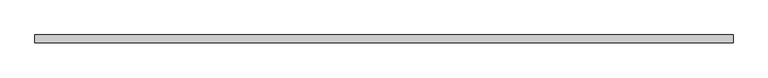
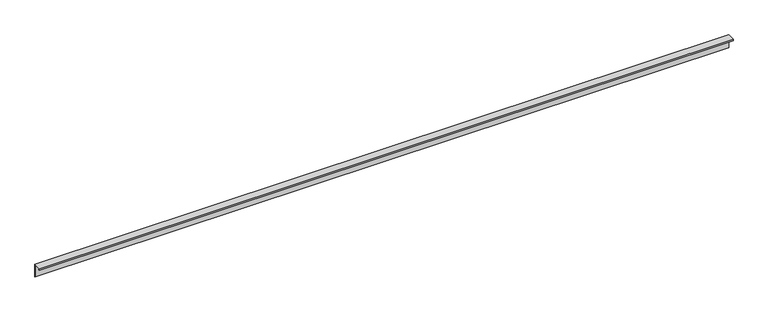
"""IFC4 building model written with IfcOpenShell, lengths in millimetres: proxy geometry, GRAVEL STOP8:GRAVEL STOP001:288466 : GRAVEL STOP8:GRAVEL STOP001:288466."""

from ifc_helpers import new_model, si_unit, frame, origin, place, context, project, spatial, polyline, outline, extrude, source, transform, mapped, element, save


def generic_models_99f10993(model_context):
    return source(origin(), model_context, "Body", "SweptSolid", [
        extrude(outline(polyline([(-5282.2354264, 40173.8996087), (-5282.2354264, 40210.7296087), (-5301.9204264, 40210.7296087), (-5301.9204264, 40208.5198087), (-5300.18797, 40208.5198087), (-5300.18797, 40207.2498087), (-5303.1904264, 40207.2498087), (-5303.1904264, 40211.9996087), (-5280.9654264, 40211.9996087), (-5280.9654264, 40173.8996087), (-5282.2354264, 40173.8996087)])), frame((17159.7769925, 0.0, 0.0), z_axis=(1.0, 0.0, 0.0), x_axis=(0.0, 1.0, 0.0)), (0.0, 0.0, 1.0), 2000.25),
    ])


if __name__ == "__main__":
    model = new_model("IFC4")
    model_context = context("Model", 3, world=origin())
    ifc_project = project(units=[si_unit("LENGTHUNIT", "METRE", prefix="MILLI")], contexts=[model_context])
    site = spatial("IfcSite", under=ifc_project)
    building = spatial("IfcBuilding", under=site)
    placement = place(None, origin())
    generic_models_shape = generic_models_99f10993(model_context)
    element("IfcBuildingElementProxy", 1, Name="GRAVEL STOP8:GRAVEL STOP001:288466 : GRAVEL STOP8:GRAVEL STOP001:288466", ObjectType="GRAVEL STOP8:GRAVEL STOP001:288466 : GRAVEL STOP8:GRAVEL STOP001:288466", at=placement, inside=building, context=model_context, shape_type="MappedRepresentation", body=[
        mapped(generic_models_shape, transform((0.0, 0.0, 0.0), x_axis=(1.0, 0.0, 0.0), y_axis=(0.0, 1.0, 0.0), z_axis=(0.0, 0.0, 1.0))),
    ])
    save(model, "model.ifc")

# Revit data of these elements
# Type "GRAVEL STOP8:GRAVEL STOP001:288466 : GRAVEL STOP8:GRAVEL STOP001:288466"
#   NameOverride = "GRAVEL STOP8:GRAVEL STOP001:288466"
#   ObjectTypeOverride = "GRAVEL STOP8:GRAVEL STOP001"
#   Reference = "GRAVEL STOP001"
#   Category = "Generic Models"
#   Tag = "288466"
# Element 1 (IfcBuildingElementProxy, "GRAVEL STOP8:GRAVEL STOP001:288466 : GRAVEL STOP8:GRAVEL STOP001:288466")
#   Materials on its faces: "COPPER STUCCO J BEAD"
# Materials
#   "COPPER STUCCO J BEAD": class "Unassigned", colour RGB 251 232 155, transparency 0, Cost = 0
